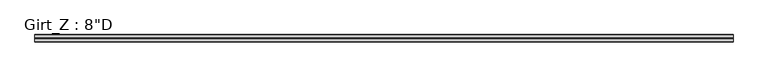
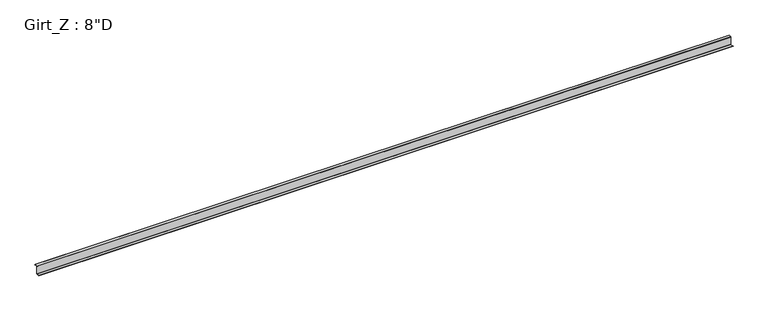
"""IFC4 building model written with IfcOpenShell, lengths in millimetres: beam geometry."""

import ifcopenshell
import ifcopenshell.guid

model = None  # the IFC model being written
_history = None  # IfcOwnerHistory: only IFC2X3 demands one
_inside = {}  # id of a spatial element -> (the spatial element, [elements in it])
_under = {}  # id of a project, library or spatial element -> (it, [spatial elements below it])
_declared = {}  # id of a project -> (the project, [libraries it declares])
_typed = {}  # id of a type object -> (the type object, [elements of that type])
_made_of = {}  # id of a material, layer set ... -> (it, [elements and type objects made of it])


def new_model(schema):
    """Start an empty IFC model of exactly this schema.

    Asked for "IFC4X3", IfcOpenShell would pick the latest addendum, in which some entities
    have other attributes; the version numbers below select the first issue.
    IFC2X3 requires an IfcOwnerHistory on every rooted entity: one is made here for all.
    """
    global model, _history
    if schema == "IFC4X3":
        model = ifcopenshell.file(schema_version=(4, 3, 0, 0))
    else:
        model = ifcopenshell.file(schema=schema)
    _inside.clear()
    _under.clear()
    _declared.clear()
    _typed.clear()
    _made_of.clear()
    _history = None
    if model.schema == "IFC2X3":
        org = make("IfcOrganization", Name="unknown")
        user = make(
            "IfcPersonAndOrganization",
            ThePerson=make("IfcPerson", FamilyName="unknown"),
            TheOrganization=org,
        )
        app = make(
            "IfcApplication",
            ApplicationDeveloper=org,
            Version="unknown",
            ApplicationFullName="unknown",
            ApplicationIdentifier="unknown",
        )
        _history = make(
            "IfcOwnerHistory",
            OwningUser=user,
            OwningApplication=app,
            ChangeAction="ADDED",
            CreationDate=0,
        )
    return model


def make(cls, **values):
    """One entity of the class cls with the attributes given. An attribute that is None is left unset."""
    return model.create_entity(
        cls, **{name: value for name, value in values.items() if value is not None}
    )


def rooted(cls, **values):
    """An entity with a GlobalId (a new one), such as an element, a storey or a relation."""
    return make(cls, GlobalId=ifcopenshell.guid.new(), OwnerHistory=_history, **values)


def si_unit(unit_type, name, prefix=None):
    """IfcSIUnit, for example si_unit("LENGTHUNIT", "METRE", prefix="MILLI")."""
    return make("IfcSIUnit", UnitType=unit_type, Prefix=prefix, Name=name)


def assignment(units):
    """IfcUnitAssignment: the units of a project."""
    return None if units is None else make("IfcUnitAssignment", Units=units)


def point(xyz):
    """IfcCartesianPoint."""
    return None if xyz is None else make("IfcCartesianPoint", Coordinates=xyz)


def direction(xyz):
    """IfcDirection."""
    return None if xyz is None else make("IfcDirection", DirectionRatios=xyz)


def frame(location, z_axis=None, x_axis=None):
    """IfcAxis2Placement3D, a coordinate frame: its origin and axes. An axis left out is left unset."""
    return make(
        "IfcAxis2Placement3D",
        Location=point(location),
        Axis=direction(z_axis),
        RefDirection=direction(x_axis),
    )


def frame_2d(location, x_axis=None):
    """IfcAxis2Placement2D, a coordinate frame in the plane: its origin and x axis."""
    return make(
        "IfcAxis2Placement2D", Location=point(location), RefDirection=direction(x_axis)
    )


def origin():
    """The frame at (0, 0, 0) with its axes left unset."""
    return frame((0.0, 0.0, 0.0))


def place(relative_to, where):
    """IfcLocalPlacement: puts the frame where relative to a parent placement (None: the world)."""
    return make(
        "IfcLocalPlacement", PlacementRelTo=relative_to, RelativePlacement=where
    )


def context(
    kind, dimensions, precision=None, world=None, true_north=None, identifier=None
):
    """IfcGeometricRepresentationContext, for example the 3D "Model" context."""
    return make(
        "IfcGeometricRepresentationContext",
        ContextIdentifier=identifier,
        ContextType=kind,
        CoordinateSpaceDimension=dimensions,
        Precision=precision,
        WorldCoordinateSystem=world,
        TrueNorth=true_north,
    )


def project(units=None, contexts=None):
    """IfcProject with its units and contexts."""
    return rooted(
        "IfcProject",
        Name="project",
        RepresentationContexts=contexts,
        UnitsInContext=assignment(units),
    )


def spatial(cls, under=None, at=None, **own):
    """A site, building, storey or space (cls), placed at a placement, below another one or the project."""
    s = rooted(cls, ObjectPlacement=at, **own)
    if under is not None:
        _under.setdefault(under.id(), (under, []))[1].append(s)
    return s


def polyline(points):
    """IfcPolyline through the points."""
    return make("IfcPolyline", Points=[point(p) for p in points])


def circle_curve(where, radius):
    """IfcCircle in the frame where."""
    return make("IfcCircle", Position=where, Radius=radius)


def trimmed(basis, trim1, trim2, sense, master):
    """IfcTrimmedCurve: the piece of a basis curve between two trims."""
    return make(
        "IfcTrimmedCurve",
        BasisCurve=basis,
        Trim1=trim1,
        Trim2=trim2,
        SenseAgreement=sense,
        MasterRepresentation=master,
    )


def segment(curve, same_sense, transition):
    """IfcCompositeCurveSegment."""
    return make(
        "IfcCompositeCurveSegment",
        Transition=transition,
        SameSense=same_sense,
        ParentCurve=curve,
    )


def composite_curve(segments, self_intersect=None):
    """IfcCompositeCurve: segments joined end to end."""
    return make("IfcCompositeCurve", Segments=segments, SelfIntersect=self_intersect)


def outline(outer, holes=None, kind="AREA"):
    """IfcArbitraryClosedProfileDef: a profile drawn as a closed curve; with holes, ...WithVoids."""
    if holes is None:
        return make("IfcArbitraryClosedProfileDef", ProfileType=kind, OuterCurve=outer)
    return make(
        "IfcArbitraryProfileDefWithVoids",
        ProfileType=kind,
        OuterCurve=outer,
        InnerCurves=holes,
    )


def extrude(swept, where, along, depth):
    """IfcExtrudedAreaSolid: the profile swept, set in the frame where, extruded along a direction by depth."""
    return make(
        "IfcExtrudedAreaSolid",
        SweptArea=swept,
        Position=where,
        ExtrudedDirection=direction(along),
        Depth=depth,
    )


def shape(context_of_items, identifier, shape_type, items):
    """IfcShapeRepresentation: the items that make up one representation, for example the "Body"."""
    return make(
        "IfcShapeRepresentation",
        ContextOfItems=context_of_items,
        RepresentationIdentifier=identifier,
        RepresentationType=shape_type,
        Items=items,
    )


def source(mapping_origin, context_of_items, identifier, shape_type, items):
    """IfcRepresentationMap: a shape defined once, which mapped items show again and again."""
    return make(
        "IfcRepresentationMap",
        MappingOrigin=mapping_origin,
        MappedRepresentation=shape(context_of_items, identifier, shape_type, items),
    )


def transform(
    local_origin,
    x_axis=None,
    y_axis=None,
    z_axis=None,
    scale=None,
    scale2=None,
    scale3=None,
    uniform=True,
):
    """IfcCartesianTransformationOperator3D, or its non-uniform kind. x_axis, y_axis, z_axis: its Axis1, 2, 3."""
    if uniform:
        return make(
            "IfcCartesianTransformationOperator3D",
            Axis1=direction(x_axis),
            Axis2=direction(y_axis),
            LocalOrigin=point(local_origin),
            Scale=scale,
            Axis3=direction(z_axis),
        )
    return make(
        "IfcCartesianTransformationOperator3DnonUniform",
        Axis1=direction(x_axis),
        Axis2=direction(y_axis),
        LocalOrigin=point(local_origin),
        Scale=scale,
        Axis3=direction(z_axis),
        Scale2=scale2,
        Scale3=scale3,
    )


def mapped(mapping_source, mapping_target):
    """IfcMappedItem: shows the shape of a source again, moved by a transform."""
    return make(
        "IfcMappedItem", MappingSource=mapping_source, MappingTarget=mapping_target
    )


def made_of(thing, what):
    """Note that an element or type object is made of a material, layer set ...; save() writes the relation."""
    if what is not None:
        _made_of.setdefault(what.id(), (what, []))[1].append(thing)
    return thing


def element(
    cls,
    number,
    at=None,
    inside=None,
    cuts=None,
    type_object=None,
    material=None,
    context=None,
    identifier="Body",
    shape_type=None,
    held_by="IfcProductDefinitionShape",
    body=None,
    shapes=None,
    **own,
):
    """One element of the class cls, such as IfcWall. Its Tag is "e" and its number.

    at: its placement. inside: the storey or other place that contains it. cuts: it is an
    opening in that element (IfcRelVoidsElement). A single representation is given by context,
    identifier, shape_type and body (its items); several are given by shapes. held_by: the class
    of the entity that holds the representations. save() writes the other relations.
    """
    e = rooted(cls, Tag="e%d" % number, ObjectPlacement=at, **own)
    if body is not None:
        shapes = [shape(context, identifier, shape_type, body)]
    if shapes is not None:
        e.Representation = make(held_by, Representations=shapes)
    if inside is not None:
        _inside.setdefault(inside.id(), (inside, []))[1].append(e)
    if cuts is not None:
        rooted(
            "IfcRelVoidsElement", RelatingBuildingElement=cuts, RelatedOpeningElement=e
        )
    if type_object is not None:
        _typed.setdefault(type_object.id(), (type_object, []))[1].append(e)
    return made_of(e, material)


def aggregate(whole, parts):
    """IfcRelAggregates: a whole, such as a stair, and the parts it consists of."""
    return rooted("IfcRelAggregates", RelatingObject=whole, RelatedObjects=parts)


def save(model, path):
    """Write the relations noted so far, then the file.

    IfcRelAggregates (storeys below a building ...), IfcRelContainedInSpatialStructure (elements
    in a storey), IfcRelDefinesByType, IfcRelAssociatesMaterial and IfcRelDeclares: one each for
    every whole, place, type object, material and project.
    """
    for whole, parts in _under.values():
        aggregate(whole, parts)
    for where, things in _inside.values():
        rooted(
            "IfcRelContainedInSpatialStructure",
            RelatedElements=things,
            RelatingStructure=where,
        )
    for kind, things in _typed.values():
        rooted("IfcRelDefinesByType", RelatedObjects=things, RelatingType=kind)
    for what, things in _made_of.values():
        rooted("IfcRelAssociatesMaterial", RelatedObjects=things, RelatingMaterial=what)
    for by, libraries in _declared.values():
        rooted("IfcRelDeclares", RelatingContext=by, RelatedDefinitions=libraries)
    model.write(path)


def beam_27ad1bc1(model_context):
    return source(origin(), model_context, "Body", "SweptSolid", [
        extrude(outline(composite_curve([segment(polyline([(77.9859375, 101.6), (90.2310415, 87.0068534), (88.1028742, 85.221109), (76.6904765, 98.821875), (3.3005807, 98.821875)]), True, "CONTINUOUS"), segment(trimmed(circle_curve(frame_2d((3.3741066, 96.8381931)), 1.9850441), [point((3.3005807, 98.821875))], [point((1.3890625, 96.8381931))], True, "CARTESIAN"), True, "CONTINUOUS"), segment(polyline([(1.3890625, 96.8381931), (1.3890625, -101.6), (-84.3359375, -101.6), (-96.5810415, -87.0068534), (-94.4528742, -85.221109), (-83.0404765, -98.821875), (-3.2694106, -98.821875)]), True, "CONTINUOUS"), segment(trimmed(circle_curve(frame_2d((-3.3748024, -96.8389339)), 1.9857399), [point((-3.2694106, -98.821875))], [point((-1.3890625, -96.8389339))], True, "CARTESIAN"), True, "CONTINUOUS"), segment(polyline([(-1.3890625, -96.8389339), (-1.3890625, 96.8375)]), True, "CONTINUOUS"), segment(trimmed(circle_curve(frame_2d((3.3734375, 96.8375)), 4.7625), [point((-1.3890625, 96.8375))], [point((3.3734375, 101.6))], False, "CARTESIAN"), True, "CONTINUOUS"), segment(polyline([(3.3734375, 101.6), (77.9859375, 101.6)]), True, "CONTINUOUS")], self_intersect=False)), frame((-8812.2125, 0.0, 0.0), z_axis=(1.0, 0.0, 0.0), x_axis=(0.0, 1.0, 0.0)), (0.0, 0.0, 1.0), 17570.45),
    ])


if __name__ == "__main__":
    model = new_model("IFC4")
    model_context = context("Model", 3, world=origin())
    ifc_project = project(units=[si_unit("LENGTHUNIT", "METRE", prefix="MILLI")], contexts=[model_context])
    site = spatial("IfcSite", under=ifc_project)
    building = spatial("IfcBuilding", under=site)
    placement = place(None, origin())
    beam_shape = beam_27ad1bc1(model_context)
    element("IfcBeam", 1, ObjectType="Girt_Z : 8\"D", at=placement, inside=building, context=model_context, shape_type="MappedRepresentation", body=[
        mapped(beam_shape, transform((0.0, 0.0, 0.0), x_axis=(1.0, 0.0, 0.0), y_axis=(0.0, 1.0, 0.0), z_axis=(0.0, 0.0, 1.0))),
    ])
    save(model, "model.ifc")

# Revit data of these elements
# Type "Girt_Z : 8\"D"
#   half leg = 0' - 1 11/16"
#   Web_Thickness = 0' - 0 7/64"
#   Length [instance default] = 10' - 0"
#   Leg_2 = 0' - 3 3/8"
#   Leg_1 = 0' - 3 1/8"
#   Height = 0' - 8"
#   Structural Material [instance default] = none
